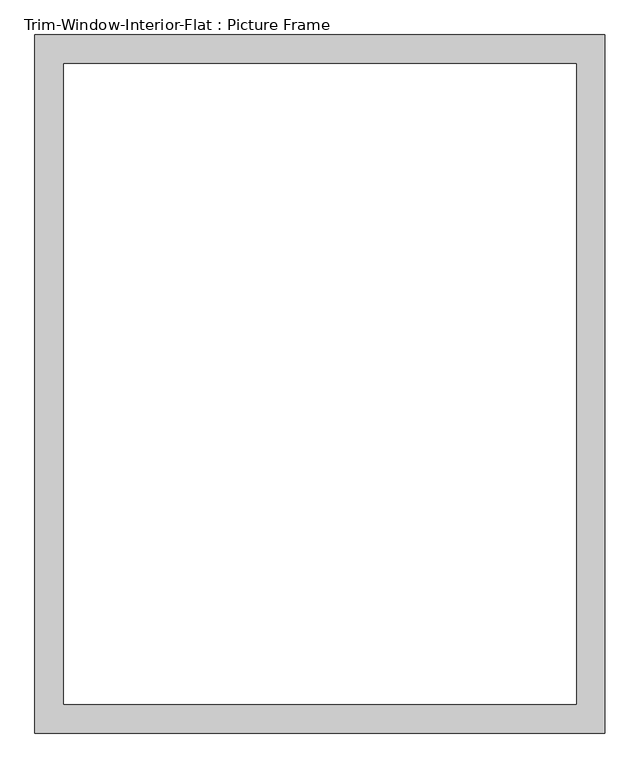
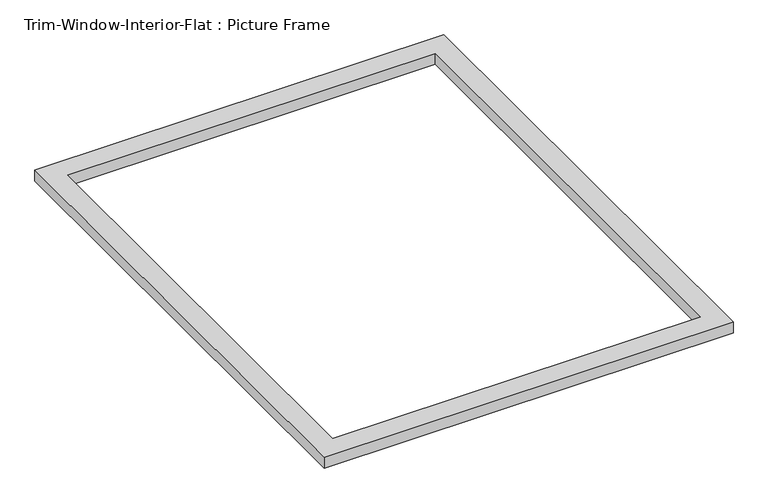
"""IFC4 building model written with IfcOpenShell, lengths in millimetres: proxy geometry, Trim-Window-Interior-Flat : Picture Frame."""

import ifcopenshell
import ifcopenshell.guid

model = None  # the IFC model being written
_history = None  # IfcOwnerHistory: only IFC2X3 demands one
_inside = {}  # id of a spatial element -> (the spatial element, [elements in it])
_under = {}  # id of a project, library or spatial element -> (it, [spatial elements below it])
_declared = {}  # id of a project -> (the project, [libraries it declares])
_typed = {}  # id of a type object -> (the type object, [elements of that type])
_made_of = {}  # id of a material, layer set ... -> (it, [elements and type objects made of it])


def new_model(schema):
    """Start an empty IFC model of exactly this schema.

    Asked for "IFC4X3", IfcOpenShell would pick the latest addendum, in which some entities
    have other attributes; the version numbers below select the first issue.
    IFC2X3 requires an IfcOwnerHistory on every rooted entity: one is made here for all.
    """
    global model, _history
    if schema == "IFC4X3":
        model = ifcopenshell.file(schema_version=(4, 3, 0, 0))
    else:
        model = ifcopenshell.file(schema=schema)
    _inside.clear()
    _under.clear()
    _declared.clear()
    _typed.clear()
    _made_of.clear()
    _history = None
    if model.schema == "IFC2X3":
        org = make("IfcOrganization", Name="unknown")
        user = make(
            "IfcPersonAndOrganization",
            ThePerson=make("IfcPerson", FamilyName="unknown"),
            TheOrganization=org,
        )
        app = make(
            "IfcApplication",
            ApplicationDeveloper=org,
            Version="unknown",
            ApplicationFullName="unknown",
            ApplicationIdentifier="unknown",
        )
        _history = make(
            "IfcOwnerHistory",
            OwningUser=user,
            OwningApplication=app,
            ChangeAction="ADDED",
            CreationDate=0,
        )
    return model


def make(cls, **values):
    """One entity of the class cls with the attributes given. An attribute that is None is left unset."""
    return model.create_entity(
        cls, **{name: value for name, value in values.items() if value is not None}
    )


def rooted(cls, **values):
    """An entity with a GlobalId (a new one), such as an element, a storey or a relation."""
    return make(cls, GlobalId=ifcopenshell.guid.new(), OwnerHistory=_history, **values)


def si_unit(unit_type, name, prefix=None):
    """IfcSIUnit, for example si_unit("LENGTHUNIT", "METRE", prefix="MILLI")."""
    return make("IfcSIUnit", UnitType=unit_type, Prefix=prefix, Name=name)


def assignment(units):
    """IfcUnitAssignment: the units of a project."""
    return None if units is None else make("IfcUnitAssignment", Units=units)


def point(xyz):
    """IfcCartesianPoint."""
    return None if xyz is None else make("IfcCartesianPoint", Coordinates=xyz)


def direction(xyz):
    """IfcDirection."""
    return None if xyz is None else make("IfcDirection", DirectionRatios=xyz)


def frame(location, z_axis=None, x_axis=None):
    """IfcAxis2Placement3D, a coordinate frame: its origin and axes. An axis left out is left unset."""
    return make(
        "IfcAxis2Placement3D",
        Location=point(location),
        Axis=direction(z_axis),
        RefDirection=direction(x_axis),
    )


def origin():
    """The frame at (0, 0, 0) with its axes left unset."""
    return frame((0.0, 0.0, 0.0))


def origin_with_axes():
    """The frame at (0, 0, 0) with the z axis (0, 0, 1) and the x axis (1, 0, 0) written out."""
    return frame((0.0, 0.0, 0.0), z_axis=(0.0, 0.0, 1.0), x_axis=(1.0, 0.0, 0.0))


def place(relative_to, where):
    """IfcLocalPlacement: puts the frame where relative to a parent placement (None: the world)."""
    return make(
        "IfcLocalPlacement", PlacementRelTo=relative_to, RelativePlacement=where
    )


def context(
    kind, dimensions, precision=None, world=None, true_north=None, identifier=None
):
    """IfcGeometricRepresentationContext, for example the 3D "Model" context."""
    return make(
        "IfcGeometricRepresentationContext",
        ContextIdentifier=identifier,
        ContextType=kind,
        CoordinateSpaceDimension=dimensions,
        Precision=precision,
        WorldCoordinateSystem=world,
        TrueNorth=true_north,
    )


def project(units=None, contexts=None):
    """IfcProject with its units and contexts."""
    return rooted(
        "IfcProject",
        Name="project",
        RepresentationContexts=contexts,
        UnitsInContext=assignment(units),
    )


def spatial(cls, under=None, at=None, **own):
    """A site, building, storey or space (cls), placed at a placement, below another one or the project."""
    s = rooted(cls, ObjectPlacement=at, **own)
    if under is not None:
        _under.setdefault(under.id(), (under, []))[1].append(s)
    return s


def polyline(points):
    """IfcPolyline through the points."""
    return make("IfcPolyline", Points=[point(p) for p in points])


def outline(outer, holes=None, kind="AREA"):
    """IfcArbitraryClosedProfileDef: a profile drawn as a closed curve; with holes, ...WithVoids."""
    if holes is None:
        return make("IfcArbitraryClosedProfileDef", ProfileType=kind, OuterCurve=outer)
    return make(
        "IfcArbitraryProfileDefWithVoids",
        ProfileType=kind,
        OuterCurve=outer,
        InnerCurves=holes,
    )


def extrude(swept, where, along, depth):
    """IfcExtrudedAreaSolid: the profile swept, set in the frame where, extruded along a direction by depth."""
    return make(
        "IfcExtrudedAreaSolid",
        SweptArea=swept,
        Position=where,
        ExtrudedDirection=direction(along),
        Depth=depth,
    )


def shape(context_of_items, identifier, shape_type, items):
    """IfcShapeRepresentation: the items that make up one representation, for example the "Body"."""
    return make(
        "IfcShapeRepresentation",
        ContextOfItems=context_of_items,
        RepresentationIdentifier=identifier,
        RepresentationType=shape_type,
        Items=items,
    )


def source(mapping_origin, context_of_items, identifier, shape_type, items):
    """IfcRepresentationMap: a shape defined once, which mapped items show again and again."""
    return make(
        "IfcRepresentationMap",
        MappingOrigin=mapping_origin,
        MappedRepresentation=shape(context_of_items, identifier, shape_type, items),
    )


def transform(
    local_origin,
    x_axis=None,
    y_axis=None,
    z_axis=None,
    scale=None,
    scale2=None,
    scale3=None,
    uniform=True,
):
    """IfcCartesianTransformationOperator3D, or its non-uniform kind. x_axis, y_axis, z_axis: its Axis1, 2, 3."""
    if uniform:
        return make(
            "IfcCartesianTransformationOperator3D",
            Axis1=direction(x_axis),
            Axis2=direction(y_axis),
            LocalOrigin=point(local_origin),
            Scale=scale,
            Axis3=direction(z_axis),
        )
    return make(
        "IfcCartesianTransformationOperator3DnonUniform",
        Axis1=direction(x_axis),
        Axis2=direction(y_axis),
        LocalOrigin=point(local_origin),
        Scale=scale,
        Axis3=direction(z_axis),
        Scale2=scale2,
        Scale3=scale3,
    )


def mapped(mapping_source, mapping_target):
    """IfcMappedItem: shows the shape of a source again, moved by a transform."""
    return make(
        "IfcMappedItem", MappingSource=mapping_source, MappingTarget=mapping_target
    )


def made_of(thing, what):
    """Note that an element or type object is made of a material, layer set ...; save() writes the relation."""
    if what is not None:
        _made_of.setdefault(what.id(), (what, []))[1].append(thing)
    return thing


def element(
    cls,
    number,
    at=None,
    inside=None,
    cuts=None,
    type_object=None,
    material=None,
    context=None,
    identifier="Body",
    shape_type=None,
    held_by="IfcProductDefinitionShape",
    body=None,
    shapes=None,
    **own,
):
    """One element of the class cls, such as IfcWall. Its Tag is "e" and its number.

    at: its placement. inside: the storey or other place that contains it. cuts: it is an
    opening in that element (IfcRelVoidsElement). A single representation is given by context,
    identifier, shape_type and body (its items); several are given by shapes. held_by: the class
    of the entity that holds the representations. save() writes the other relations.
    """
    e = rooted(cls, Tag="e%d" % number, ObjectPlacement=at, **own)
    if body is not None:
        shapes = [shape(context, identifier, shape_type, body)]
    if shapes is not None:
        e.Representation = make(held_by, Representations=shapes)
    if inside is not None:
        _inside.setdefault(inside.id(), (inside, []))[1].append(e)
    if cuts is not None:
        rooted(
            "IfcRelVoidsElement", RelatingBuildingElement=cuts, RelatedOpeningElement=e
        )
    if type_object is not None:
        _typed.setdefault(type_object.id(), (type_object, []))[1].append(e)
    return made_of(e, material)


def aggregate(whole, parts):
    """IfcRelAggregates: a whole, such as a stair, and the parts it consists of."""
    return rooted("IfcRelAggregates", RelatingObject=whole, RelatedObjects=parts)


def save(model, path):
    """Write the relations noted so far, then the file.

    IfcRelAggregates (storeys below a building ...), IfcRelContainedInSpatialStructure (elements
    in a storey), IfcRelDefinesByType, IfcRelAssociatesMaterial and IfcRelDeclares: one each for
    every whole, place, type object, material and project.
    """
    for whole, parts in _under.values():
        aggregate(whole, parts)
    for where, things in _inside.values():
        rooted(
            "IfcRelContainedInSpatialStructure",
            RelatedElements=things,
            RelatingStructure=where,
        )
    for kind, things in _typed.values():
        rooted("IfcRelDefinesByType", RelatedObjects=things, RelatingType=kind)
    for what, things in _made_of.values():
        rooted("IfcRelAssociatesMaterial", RelatedObjects=things, RelatingMaterial=what)
    for by, libraries in _declared.values():
        rooted("IfcRelDeclares", RelatingContext=by, RelatedDefinitions=libraries)
    model.write(path)


def trim_window_interior_flat_picture_frame_7cb3e35f(model_context):
    return source(origin(), model_context, "Body", "SweptSolid", [
        extrude(outline(polyline([(565.15, -44.45), (-565.15, -44.45), (-565.15, 1339.85), (565.15, 1339.85), (565.15, -44.45)]), holes=[polyline([(508.0, 12.7), (508.0, 1282.7), (-508.0, 1282.7), (-508.0, 12.7), (508.0, 12.7)])]), origin_with_axes(), (0.0, 0.0, 1.0), 31.75),
    ])


if __name__ == "__main__":
    model = new_model("IFC4")
    model_context = context("Model", 3, world=origin())
    ifc_project = project(units=[si_unit("LENGTHUNIT", "METRE", prefix="MILLI")], contexts=[model_context])
    site = spatial("IfcSite", under=ifc_project)
    building = spatial("IfcBuilding", under=site)
    placement = place(None, origin())
    trim_window_interior_flat_picture_frame_shape = trim_window_interior_flat_picture_frame_7cb3e35f(model_context)
    element("IfcBuildingElementProxy", 1, Name="Trim-Window-Interior-Flat : Picture Frame", ObjectType="Trim-Window-Interior-Flat : Picture Frame", at=placement, inside=building, context=model_context, shape_type="MappedRepresentation", body=[
        mapped(trim_window_interior_flat_picture_frame_shape, transform((0.0, 0.0, 0.0), x_axis=(1.0, 0.0, 0.0), y_axis=(0.0, 1.0, 0.0), z_axis=(0.0, 0.0, 1.0))),
    ])
    save(model, "model.ifc")

# Revit data of these elements
# Type "Trim-Window-Interior-Flat : Picture Frame"
#   Trim Thickness_Picture Frame = 0' - 1 1/4"
#   Trim Width = 0' - 2 1/4"
#   Trim Thickness_with Sill = 0' - 0 3/4"
#   Sill Thickness = 0' - 1 1/4"
#   Opening Width [instance default] = 2' - 0"
#   Opening Height [instance default] = 3' - 0"
#   Default Elevation = 4' - 0"
#   Sill = no
#   Picture Frame = yes
#   Trim Material [instance default] = none
# Element 1 (IfcBuildingElementProxy, "Trim-Window-Interior-Flat : Picture Frame")
#   Opening Width = 3' - 5"
#   Opening Height = 4' - 3"
#   Trim Material = Wood - Stained
#   Materials on its faces: "Wood - Stained"
# Materials
#   "Wood - Stained": class "Wood", colour RGB 224 178 126, transparency 0, Cost = 0
